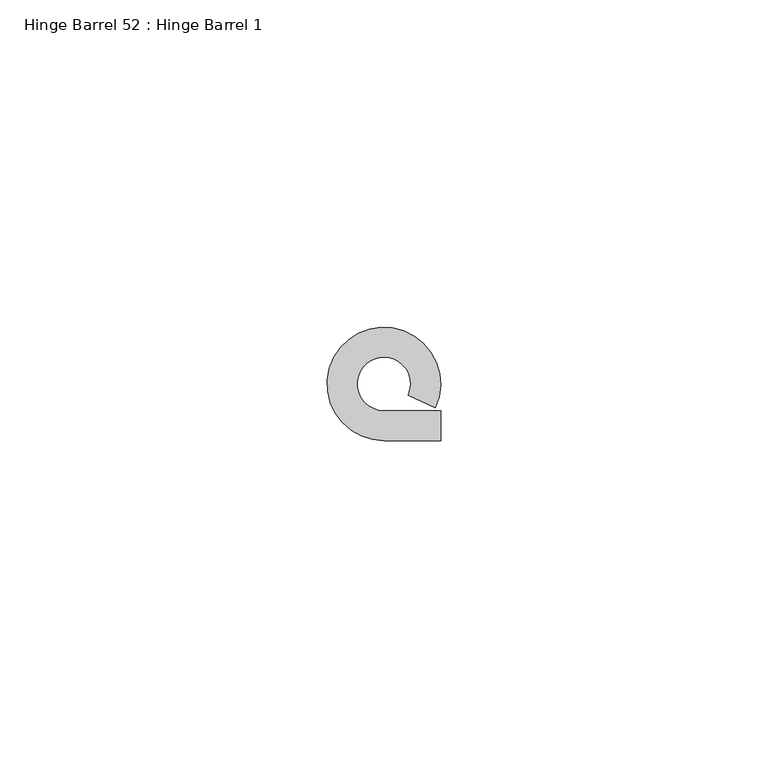
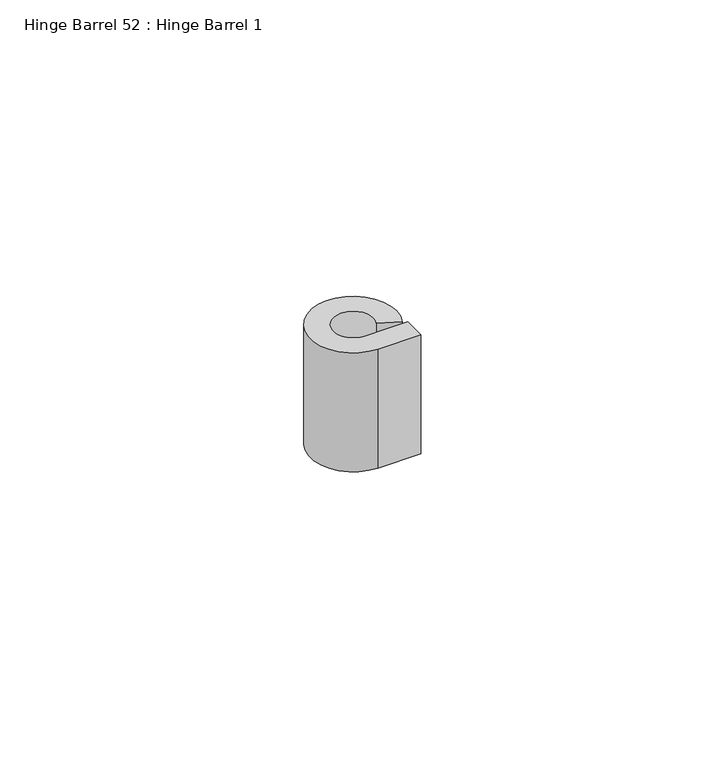
"""IFC4 building model written with IfcOpenShell, lengths in millimetres: proxy geometry, Hinge Barrel 52 : Hinge Barrel 1."""

from ifc_helpers import new_model, si_unit, point, frame, frame_2d, origin, place, context, project, spatial, polyline, circle_curve, trimmed, segment, composite_curve, outline, extrude, source, transform, mapped, element, save


def hinge_barrel_52_hinge_barrel_1_6a8bf010(model_context):
    return source(origin(), model_context, "Body", "SweptSolid", [
        extrude(outline(composite_curve([segment(polyline([(587323.2214739, -534104.7943841), (587327.7934739, -534104.7943841), (587327.7934739, -534109.3584466), (587319.1320739, -534109.3584466)]), True, "CONTINUOUS"), segment(trimmed(circle_curve(frame_2d((587319.1320739, -534100.7049841)), 8.6534625), [point((587319.1320739, -534109.3584466))], [point((587326.986084, -534104.3377433))], False, "CARTESIAN"), True, "CONTINUOUS"), segment(polyline([(587326.986084, -534104.3377433), (587322.8436736, -534102.421731)]), True, "CONTINUOUS"), segment(trimmed(circle_curve(frame_2d((587319.1320739, -534100.7049841)), 4.0894), [point((587322.8436736, -534102.421731))], [point((587319.1320739, -534104.7943841))], True, "CARTESIAN"), True, "CONTINUOUS"), segment(polyline([(587319.1320739, -534104.7943841), (587323.2214739, -534104.7943841)]), True, "CONTINUOUS")], self_intersect=False)), frame((0.0, 0.0, 1225.55), z_axis=(0.0, 0.0, 1.0), x_axis=(1.0, 0.0, 0.0)), (0.0, 0.0, 1.0), 25.4),
    ])


if __name__ == "__main__":
    model = new_model("IFC4")
    model_context = context("Model", 3, world=origin())
    ifc_project = project(units=[si_unit("LENGTHUNIT", "METRE", prefix="MILLI")], contexts=[model_context])
    site = spatial("IfcSite", under=ifc_project)
    building = spatial("IfcBuilding", under=site)
    placement = place(None, origin())
    hinge_barrel_52_hinge_barrel_1_shape = hinge_barrel_52_hinge_barrel_1_6a8bf010(model_context)
    element("IfcBuildingElementProxy", 1, Name="Hinge Barrel 52 : Hinge Barrel 1", ObjectType="Hinge Barrel 52 : Hinge Barrel 1", at=placement, inside=building, context=model_context, shape_type="MappedRepresentation", body=[
        mapped(hinge_barrel_52_hinge_barrel_1_shape, transform((0.0, 0.0, 0.0), x_axis=(1.0, 0.0, 0.0), y_axis=(0.0, 1.0, 0.0), z_axis=(0.0, 0.0, 1.0))),
    ])
    save(model, "model.ifc")

# Revit data of these elements
# Element 1 (IfcBuildingElementProxy, "Hinge Barrel 52 : Hinge Barrel 1")
#   Materials on its faces: "6\"X6\" WELD-ON STL BUTT HINGE"
# Materials
#   "6\"X6\" WELD-ON STL BUTT HINGE": class "Metal", colour RGB 189 187 185, transparency 0, Description = "Carbon steel", Cost = 0
